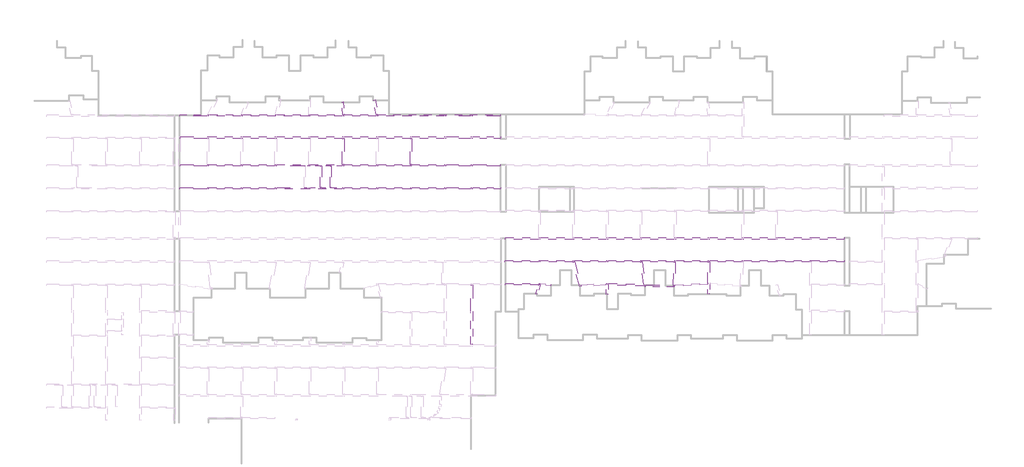
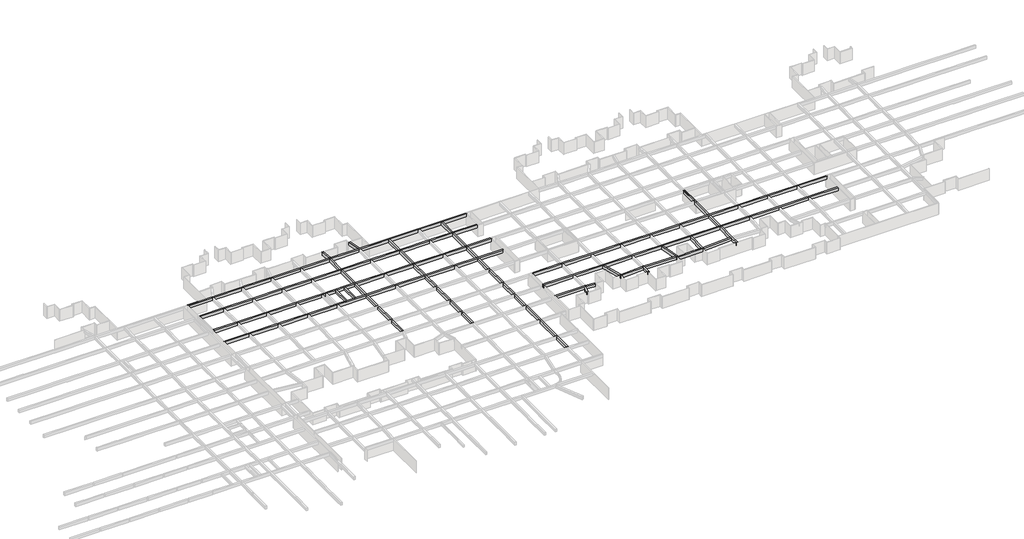
# One storey, part 14 of 16: 25 beams.
"""IFC4 building model written with IfcOpenShell, lengths in millimetres."""

from ifc_helpers import new_model, si_unit, frame, origin, place, context, project, spatial, polyline, outline, extrude, faceted_brep, element, save

model = new_model("IFC4")

# Units and contexts
model_context = context("Model", 3, world=origin())
ifc_project = project(units=[si_unit("LENGTHUNIT", "METRE", prefix="MILLI")], contexts=[model_context])

# Site, building, storey
site = spatial("IfcSite", under=ifc_project)
building = spatial("IfcBuilding", under=site)
storey = spatial("IfcBuildingStorey", under=building, Name="户型图", Elevation=0.0)

# Beams
placement = place(None, origin())
element("IfcBeam", 1, ObjectType="混凝土 - 矩形梁 : KL_beam", at=placement, inside=storey, context=model_context, shape_type="Brep", body=[
    faceted_brep([(332003.757676, -132296.8999905, 3300.0), (332003.757676, -132696.8999905, 3300.0), (332003.757676, -132696.8999905, 2500.0), (332003.757676, -132296.8999905, 2500.0), (256203.757676, -132296.8999905, 3300.0), (256203.757676, -132296.8999905, 2500.0), (256203.757676, -132696.8999905, 2500.0), (256203.757676, -132696.8999905, 3300.0), (303083.9231733, -132296.8999905, 3300.0), (302676.4364954, -132296.8999905, 3300.0), (295182.986598, -132296.8999905, 3300.0), (294781.458663, -132296.8999905, 3300.0), (287099.7203632, -132296.8999905, 3300.0), (286699.7203632, -132296.8999905, 3300.0), (279255.0563689, -132296.8999905, 3300.0), (278842.8109172, -132296.8999905, 3300.0), (271220.3376586, -132296.8999905, 3300.0), (270785.7935076, -132296.8999905, 3300.0), (263349.1220942, -132296.8999905, 3300.0), (262900.1915992, -132296.8999905, 3300.0), (262755.329592, -132696.8999905, 3300.0), (263155.329592, -132696.8999905, 3300.0), (270718.1706199, -132696.8999905, 3300.0), (271118.1706199, -132696.8999905, 3300.0), (286699.7203632, -132696.8999905, 3300.0), (287099.7203632, -132696.8999905, 3300.0), (294691.573786, -132696.8999905, 3300.0), (295091.573786, -132696.8999905, 3300.0), (302719.0558962, -132696.8999905, 3300.0), (303119.0558962, -132696.8999905, 3300.0), (310675.2880408, -132696.8999905, 3300.0), (311075.2880408, -132696.8999905, 3300.0), (318775.2880408, -132696.8999905, 3300.0), (319175.2880408, -132696.8999905, 3300.0), (325052.9173169, -132696.8999905, 3300.0), (325452.9173169, -132696.8999905, 3300.0), (262755.329592, -132696.8999905, 2500.0), (263155.329592, -132696.8999905, 2500.0), (270718.1706199, -132696.8999905, 2500.0), (271118.1706199, -132696.8999905, 2500.0), (286699.7203632, -132696.8999905, 2500.0), (287099.7203632, -132696.8999905, 2500.0), (294691.573786, -132696.8999905, 2500.0), (295091.573786, -132696.8999905, 2500.0), (302719.0558962, -132696.8999905, 2500.0), (303119.0558962, -132696.8999905, 2500.0), (310675.2880408, -132696.8999905, 2500.0), (311075.2880408, -132696.8999905, 2500.0), (318775.2880408, -132696.8999905, 2500.0), (319175.2880408, -132696.8999905, 2500.0), (325052.9173169, -132696.8999905, 2500.0), (325452.9173169, -132696.8999905, 2500.0), (262900.1915992, -132296.8999905, 2500.0), (263349.1220942, -132296.8999905, 2500.0), (270785.7935076, -132296.8999905, 2500.0), (271220.3376586, -132296.8999905, 2500.0), (278842.8109172, -132296.8999905, 2500.0), (279255.0563689, -132296.8999905, 2500.0), (286699.7203632, -132296.8999905, 2500.0), (287099.7203632, -132296.8999905, 2500.0), (294781.458663, -132296.8999905, 2500.0), (295182.986598, -132296.8999905, 2500.0), (302676.4364954, -132296.8999905, 2500.0), (303083.9231733, -132296.8999905, 2500.0)], [[[0, 1, 2, 3]], [[4, 5, 6, 7]], [[1, 0, 8, 9, 10, 11, 12, 13, 14, 15, 16, 17, 18, 19, 4, 7, 20, 21, 22, 23, 24, 25, 26, 27, 28, 29, 30, 31, 32, 33, 34, 35]], [[2, 1, 35, 34, 33, 32, 31, 30, 29, 28, 27, 26, 25, 24, 23, 22, 21, 20, 7, 6, 36, 37, 38, 39, 40, 41, 42, 43, 44, 45, 46, 47, 48, 49, 50, 51]], [[3, 2, 51, 50, 49, 48, 47, 46, 45, 44, 43, 42, 41, 40, 39, 38, 37, 36, 6, 5, 52, 53, 54, 55, 56, 57, 58, 59, 60, 61, 62, 63]], [[0, 3, 63, 62, 61, 60, 59, 58, 57, 56, 55, 54, 53, 52, 5, 4, 19, 18, 17, 16, 15, 14, 13, 12, 11, 10, 9, 8]]]),
])
element("IfcBeam", 2, ObjectType="混凝土 - 矩形梁 : KL_beam", at=placement, inside=storey, context=model_context, shape_type="SweptSolid", body=[
    extrude(outline(polyline([(294521.5830468, -129326.5081051), (294920.060926, -129291.645808), (295182.986598, -132296.8999905), (294781.458663, -132296.8999905), (294521.5830468, -129326.5081051)])), frame((0.0, 0.0, 2500.0), z_axis=(0.0, 0.0, 1.0), x_axis=(1.0, 0.0, 0.0)), (0.0, 0.0, 1.0), 800.0),
])
element("IfcBeam", 3, ObjectType="混凝土 - 矩形梁 : KL_beam", at=placement, inside=storey, context=model_context, shape_type="SweptSolid", body=[
    extrude(outline(polyline([(302016.7371766, -128903.0412108), (302409.38805, -128826.7176126), (303083.9231733, -132296.8999905), (302676.4364954, -132296.8999905), (302016.7371766, -128903.0412108)])), frame((0.0, 0.0, 2500.0), z_axis=(0.0, 0.0, 1.0), x_axis=(1.0, 0.0, 0.0)), (0.0, 0.0, 1.0), 800.0),
])
element("IfcBeam", 4, ObjectType="混凝土 - 矩形梁 : KL_beam", at=placement, inside=storey, context=model_context, shape_type="Brep", body=[
    faceted_brep([(332103.757676, -137565.7214763, 3300.0), (332103.757676, -137965.7214763, 3300.0), (332103.757676, -137965.7214763, 2500.0), (332103.757676, -137565.7214763, 2500.0), (325452.9173169, -137565.7214763, 3300.0), (325052.9173169, -137565.7214763, 3300.0), (319175.2880408, -137565.7214763, 3300.0), (318775.2880408, -137565.7214763, 3300.0), (311075.2880408, -137565.7214763, 3300.0), (310675.2880408, -137565.7214763, 3300.0), (303119.0558962, -137565.7214763, 3300.0), (302719.0558962, -137565.7214763, 3300.0), (295091.573786, -137565.7214763, 3300.0), (294691.573786, -137565.7214763, 3300.0), (287099.7203632, -137565.7214763, 3300.0), (286699.7203632, -137565.7214763, 3300.0), (279139.6845219, -137565.7214763, 3300.0), (278739.6845219, -137565.7214763, 3300.0), (271118.1706199, -137565.7214763, 3300.0), (270718.1706199, -137565.7214763, 3300.0), (263155.329592, -137565.7214763, 3300.0), (262755.329592, -137565.7214763, 3300.0), (256403.757676, -137565.7214763, 3300.0), (256403.757676, -137965.7214763, 3300.0), (262755.329592, -137965.7214763, 3300.0), (263155.329592, -137965.7214763, 3300.0), (270718.1706199, -137965.7214763, 3300.0), (271118.1706199, -137965.7214763, 3300.0), (278739.6845219, -137965.7214763, 3300.0), (279139.6845219, -137965.7214763, 3300.0), (286699.7203632, -137965.7214763, 3300.0), (287099.7203632, -137965.7214763, 3300.0), (294691.573786, -137965.7214763, 3300.0), (295091.573786, -137965.7214763, 3300.0), (302719.0558962, -137965.7214763, 3300.0), (303119.0558962, -137965.7214763, 3300.0), (310675.2880408, -137965.7214763, 3300.0), (311075.2880408, -137965.7214763, 3300.0), (318775.2880408, -137965.7214763, 3300.0), (319175.2880408, -137965.7214763, 3300.0), (325052.9173169, -137965.7214763, 3300.0), (325452.9173169, -137965.7214763, 3300.0), (256403.757676, -137965.7214763, 2500.0), (262755.329592, -137965.7214763, 2500.0), (263155.329592, -137965.7214763, 2500.0), (270718.1706199, -137965.7214763, 2500.0), (271118.1706199, -137965.7214763, 2500.0), (278739.6845219, -137965.7214763, 2500.0), (279139.6845219, -137965.7214763, 2500.0), (286699.7203632, -137965.7214763, 2500.0), (287099.7203632, -137965.7214763, 2500.0), (294691.573786, -137965.7214763, 2500.0), (295091.573786, -137965.7214763, 2500.0), (302719.0558962, -137965.7214763, 2500.0), (303119.0558962, -137965.7214763, 2500.0), (310675.2880408, -137965.7214763, 2500.0), (311075.2880408, -137965.7214763, 2500.0), (318775.2880408, -137965.7214763, 2500.0), (319175.2880408, -137965.7214763, 2500.0), (325052.9173169, -137965.7214763, 2500.0), (325452.9173169, -137965.7214763, 2500.0), (256403.757676, -137565.7214763, 2500.0), (262755.329592, -137565.7214763, 2500.0), (263155.329592, -137565.7214763, 2500.0), (270718.1706199, -137565.7214763, 2500.0), (271118.1706199, -137565.7214763, 2500.0), (278739.6845219, -137565.7214763, 2500.0), (279139.6845219, -137565.7214763, 2500.0), (286699.7203632, -137565.7214763, 2500.0), (287099.7203632, -137565.7214763, 2500.0), (294691.573786, -137565.7214763, 2500.0), (295091.573786, -137565.7214763, 2500.0), (302719.0558962, -137565.7214763, 2500.0), (303119.0558962, -137565.7214763, 2500.0), (310675.2880408, -137565.7214763, 2500.0), (311075.2880408, -137565.7214763, 2500.0), (318775.2880408, -137565.7214763, 2500.0), (319175.2880408, -137565.7214763, 2500.0), (325052.9173169, -137565.7214763, 2500.0), (325452.9173169, -137565.7214763, 2500.0)], [[[0, 1, 2, 3]], [[1, 0, 4, 5, 6, 7, 8, 9, 10, 11, 12, 13, 14, 15, 16, 17, 18, 19, 20, 21, 22, 23, 24, 25, 26, 27, 28, 29, 30, 31, 32, 33, 34, 35, 36, 37, 38, 39, 40, 41]], [[2, 1, 41, 40, 39, 38, 37, 36, 35, 34, 33, 32, 31, 30, 29, 28, 27, 26, 25, 24, 23, 42, 43, 44, 45, 46, 47, 48, 49, 50, 51, 52, 53, 54, 55, 56, 57, 58, 59, 60]], [[3, 2, 60, 59, 58, 57, 56, 55, 54, 53, 52, 51, 50, 49, 48, 47, 46, 45, 44, 43, 42, 61, 62, 63, 64, 65, 66, 67, 68, 69, 70, 71, 72, 73, 74, 75, 76, 77, 78, 79]], [[0, 3, 79, 78, 77, 76, 75, 74, 73, 72, 71, 70, 69, 68, 67, 66, 65, 64, 63, 62, 61, 22, 21, 20, 19, 18, 17, 16, 15, 14, 13, 12, 11, 10, 9, 8, 7, 6, 5, 4]], [[23, 22, 61, 42]]]),
])
element("IfcBeam", 5, ObjectType="混凝土 - 矩形梁 : KL_beam", at=placement, inside=storey, context=model_context, shape_type="Brep", body=[
    faceted_brep([(332003.757676, -144125.7214763, 3300.0), (332003.757676, -144525.7214763, 3300.0), (332003.757676, -144525.7214763, 2500.0), (332003.757676, -144125.7214763, 2500.0), (325452.9173169, -144125.7214763, 3300.0), (325052.9173169, -144125.7214763, 3300.0), (319175.2880408, -144125.7214763, 3300.0), (318775.2880408, -144125.7214763, 3300.0), (311075.2880408, -144125.7214763, 3300.0), (310675.2880408, -144125.7214763, 3300.0), (303119.0558962, -144125.7214763, 3300.0), (302719.0558962, -144125.7214763, 3300.0), (295091.573786, -144125.7214763, 3300.0), (294691.573786, -144125.7214763, 3300.0), (287099.7203632, -144125.7214763, 3300.0), (286699.7203632, -144125.7214763, 3300.0), (279139.6845219, -144125.7214763, 3300.0), (278739.6845219, -144125.7214763, 3300.0), (271118.1706199, -144125.7214763, 3300.0), (270718.1706199, -144125.7214763, 3300.0), (263155.329592, -144125.7214763, 3300.0), (262755.329592, -144125.7214763, 3300.0), (256403.757676, -144125.7214763, 3300.0), (256403.757676, -144525.7214763, 3300.0), (262755.329592, -144525.7214763, 3300.0), (263155.329592, -144525.7214763, 3300.0), (270718.1706199, -144525.7214763, 3300.0), (271118.1706199, -144525.7214763, 3300.0), (278739.6845219, -144525.7214763, 3300.0), (279139.6845219, -144525.7214763, 3300.0), (285649.7203632, -144525.7214763, 3300.0), (285949.7203632, -144525.7214763, 3300.0), (286699.7203632, -144525.7214763, 3300.0), (287099.7203632, -144525.7214763, 3300.0), (289449.7203632, -144525.7214763, 3300.0), (289749.7203632, -144525.7214763, 3300.0), (291749.7203632, -144525.7214763, 3300.0), (292049.7203632, -144525.7214763, 3300.0), (294691.573786, -144525.7214763, 3300.0), (295091.573786, -144525.7214763, 3300.0), (302719.0558962, -144525.7214763, 3300.0), (303119.0558962, -144525.7214763, 3300.0), (310675.2880408, -144525.7214763, 3300.0), (311075.2880408, -144525.7214763, 3300.0), (318775.2880408, -144525.7214763, 3300.0), (319175.2880408, -144525.7214763, 3300.0), (325052.9173169, -144525.7214763, 3300.0), (325452.9173169, -144525.7214763, 3300.0), (256403.757676, -144525.7214763, 2500.0), (262755.329592, -144525.7214763, 2500.0), (263155.329592, -144525.7214763, 2500.0), (270718.1706199, -144525.7214763, 2500.0), (271118.1706199, -144525.7214763, 2500.0), (278739.6845219, -144525.7214763, 2500.0), (279139.6845219, -144525.7214763, 2500.0), (286699.7203632, -144525.7214763, 2500.0), (287099.7203632, -144525.7214763, 2500.0), (294691.573786, -144525.7214763, 2500.0), (295091.573786, -144525.7214763, 2500.0), (302719.0558962, -144525.7214763, 2500.0), (303119.0558962, -144525.7214763, 2500.0), (310675.2880408, -144525.7214763, 2500.0), (311075.2880408, -144525.7214763, 2500.0), (318775.2880408, -144525.7214763, 2500.0), (319175.2880408, -144525.7214763, 2500.0), (325052.9173169, -144525.7214763, 2500.0), (325452.9173169, -144525.7214763, 2500.0), (256403.757676, -144125.7214763, 2500.0), (262755.329592, -144125.7214763, 2500.0), (263155.329592, -144125.7214763, 2500.0), (270718.1706199, -144125.7214763, 2500.0), (271118.1706199, -144125.7214763, 2500.0), (278739.6845219, -144125.7214763, 2500.0), (279139.6845219, -144125.7214763, 2500.0), (286699.7203632, -144125.7214763, 2500.0), (287099.7203632, -144125.7214763, 2500.0), (294691.573786, -144125.7214763, 2500.0), (295091.573786, -144125.7214763, 2500.0), (302719.0558962, -144125.7214763, 2500.0), (303119.0558962, -144125.7214763, 2500.0), (310675.2880408, -144125.7214763, 2500.0), (311075.2880408, -144125.7214763, 2500.0), (318775.2880408, -144125.7214763, 2500.0), (319175.2880408, -144125.7214763, 2500.0), (325052.9173169, -144125.7214763, 2500.0), (325452.9173169, -144125.7214763, 2500.0)], [[[0, 1, 2, 3]], [[1, 0, 4, 5, 6, 7, 8, 9, 10, 11, 12, 13, 14, 15, 16, 17, 18, 19, 20, 21, 22, 23, 24, 25, 26, 27, 28, 29, 30, 31, 32, 33, 34, 35, 36, 37, 38, 39, 40, 41, 42, 43, 44, 45, 46, 47]], [[2, 1, 47, 46, 45, 44, 43, 42, 41, 40, 39, 38, 37, 36, 35, 34, 33, 32, 31, 30, 29, 28, 27, 26, 25, 24, 23, 48, 49, 50, 51, 52, 53, 54, 55, 56, 57, 58, 59, 60, 61, 62, 63, 64, 65, 66]], [[3, 2, 66, 65, 64, 63, 62, 61, 60, 59, 58, 57, 56, 55, 54, 53, 52, 51, 50, 49, 48, 67, 68, 69, 70, 71, 72, 73, 74, 75, 76, 77, 78, 79, 80, 81, 82, 83, 84, 85]], [[0, 3, 85, 84, 83, 82, 81, 80, 79, 78, 77, 76, 75, 74, 73, 72, 71, 70, 69, 68, 67, 22, 21, 20, 19, 18, 17, 16, 15, 14, 13, 12, 11, 10, 9, 8, 7, 6, 5, 4]], [[23, 22, 67, 48]]]),
])
element("IfcBeam", 6, ObjectType="混凝土 - 矩形梁 : KL_beam", at=placement, inside=storey, context=model_context, shape_type="Brep", body=[
    faceted_brep([(332103.757676, -149525.7214763, 3300.0), (332103.757676, -149925.7214763, 3300.0), (332103.757676, -149925.7214763, 2500.0), (332103.757676, -149525.7214763, 2500.0), (256203.757676, -149525.7214763, 3300.0), (256203.757676, -149525.7214763, 2500.0), (256203.757676, -149925.7214763, 2500.0), (256203.757676, -149925.7214763, 3300.0), (325452.9173169, -149525.7214763, 3300.0), (325052.9173169, -149525.7214763, 3300.0), (319175.2880408, -149525.7214763, 3300.0), (318775.2880408, -149525.7214763, 3300.0), (311075.2880408, -149525.7214763, 3300.0), (310675.2880408, -149525.7214763, 3300.0), (303119.0558962, -149525.7214763, 3300.0), (302719.0558962, -149525.7214763, 3300.0), (295091.573786, -149525.7214763, 3300.0), (294691.573786, -149525.7214763, 3300.0), (292049.7203632, -149525.7214763, 3300.0), (291749.7203632, -149525.7214763, 3300.0), (289749.7203632, -149525.7214763, 3300.0), (289449.7203632, -149525.7214763, 3300.0), (287099.7203632, -149525.7214763, 3300.0), (286699.7203632, -149525.7214763, 3300.0), (285949.7203632, -149525.7214763, 3300.0), (285649.7203632, -149525.7214763, 3300.0), (279139.6845219, -149525.7214763, 3300.0), (278739.6845219, -149525.7214763, 3300.0), (271118.1706199, -149525.7214763, 3300.0), (270718.1706199, -149525.7214763, 3300.0), (263155.329592, -149525.7214763, 3300.0), (262755.329592, -149525.7214763, 3300.0), (262755.329592, -149925.7214763, 3300.0), (263155.329592, -149925.7214763, 3300.0), (270718.1706199, -149925.7214763, 3300.0), (271118.1706199, -149925.7214763, 3300.0), (278739.6845219, -149925.7214763, 3300.0), (279139.6845219, -149925.7214763, 3300.0), (286699.7203632, -149925.7214763, 3300.0), (287099.7203632, -149925.7214763, 3300.0), (294691.573786, -149925.7214763, 3300.0), (295091.573786, -149925.7214763, 3300.0), (302719.0558962, -149925.7214763, 3300.0), (303119.0558962, -149925.7214763, 3300.0), (310675.2880408, -149925.7214763, 3300.0), (311075.2880408, -149925.7214763, 3300.0), (318775.2880408, -149925.7214763, 3300.0), (319175.2880408, -149925.7214763, 3300.0), (325052.9173169, -149925.7214763, 3300.0), (325452.9173169, -149925.7214763, 3300.0), (262755.329592, -149925.7214763, 2500.0), (263155.329592, -149925.7214763, 2500.0), (270718.1706199, -149925.7214763, 2500.0), (271118.1706199, -149925.7214763, 2500.0), (278739.6845219, -149925.7214763, 2500.0), (279139.6845219, -149925.7214763, 2500.0), (286699.7203632, -149925.7214763, 2500.0), (287099.7203632, -149925.7214763, 2500.0), (294691.573786, -149925.7214763, 2500.0), (295091.573786, -149925.7214763, 2500.0), (302719.0558962, -149925.7214763, 2500.0), (303119.0558962, -149925.7214763, 2500.0), (310675.2880408, -149925.7214763, 2500.0), (311075.2880408, -149925.7214763, 2500.0), (318775.2880408, -149925.7214763, 2500.0), (319175.2880408, -149925.7214763, 2500.0), (325052.9173169, -149925.7214763, 2500.0), (325452.9173169, -149925.7214763, 2500.0), (262755.329592, -149525.7214763, 2500.0), (263155.329592, -149525.7214763, 2500.0), (270718.1706199, -149525.7214763, 2500.0), (271118.1706199, -149525.7214763, 2500.0), (278739.6845219, -149525.7214763, 2500.0), (279139.6845219, -149525.7214763, 2500.0), (286699.7203632, -149525.7214763, 2500.0), (287099.7203632, -149525.7214763, 2500.0), (294691.573786, -149525.7214763, 2500.0), (295091.573786, -149525.7214763, 2500.0), (302719.0558962, -149525.7214763, 2500.0), (303119.0558962, -149525.7214763, 2500.0), (310675.2880408, -149525.7214763, 2500.0), (311075.2880408, -149525.7214763, 2500.0), (318775.2880408, -149525.7214763, 2500.0), (319175.2880408, -149525.7214763, 2500.0), (325052.9173169, -149525.7214763, 2500.0), (325452.9173169, -149525.7214763, 2500.0)], [[[0, 1, 2, 3]], [[4, 5, 6, 7]], [[1, 0, 8, 9, 10, 11, 12, 13, 14, 15, 16, 17, 18, 19, 20, 21, 22, 23, 24, 25, 26, 27, 28, 29, 30, 31, 4, 7, 32, 33, 34, 35, 36, 37, 38, 39, 40, 41, 42, 43, 44, 45, 46, 47, 48, 49]], [[2, 1, 49, 48, 47, 46, 45, 44, 43, 42, 41, 40, 39, 38, 37, 36, 35, 34, 33, 32, 7, 6, 50, 51, 52, 53, 54, 55, 56, 57, 58, 59, 60, 61, 62, 63, 64, 65, 66, 67]], [[3, 2, 67, 66, 65, 64, 63, 62, 61, 60, 59, 58, 57, 56, 55, 54, 53, 52, 51, 50, 6, 5, 68, 69, 70, 71, 72, 73, 74, 75, 76, 77, 78, 79, 80, 81, 82, 83, 84, 85]], [[0, 3, 85, 84, 83, 82, 81, 80, 79, 78, 77, 76, 75, 74, 73, 72, 71, 70, 69, 68, 5, 4, 31, 30, 29, 28, 27, 26, 25, 24, 23, 22, 21, 20, 19, 18, 17, 16, 15, 14, 13, 12, 11, 10, 9, 8]]]),
])
element("IfcBeam", 7, ObjectType="混凝土 - 矩形梁 : KL_beam", at=placement, inside=storey, context=model_context, shape_type="SweptSolid", body=[
    extrude(outline(polyline([(295091.573786, -166823.3600959), (294691.573786, -166823.3600959), (294691.573786, -161826.0461868), (295091.573786, -161826.0461868), (295091.573786, -166823.3600959)])), frame((0.0, 0.0, 2500.0), z_axis=(0.0, 0.0, 1.0), x_axis=(1.0, 0.0, 0.0)), (0.0, 0.0, 1.0), 800.0),
    extrude(outline(polyline([(294691.573786, -132696.8999905), (295091.573786, -132696.8999905), (295091.573786, -137565.7214763), (294691.573786, -137565.7214763), (294691.573786, -132696.8999905)])), frame((0.0, 0.0, 2500.0), z_axis=(0.0, 0.0, 1.0), x_axis=(1.0, 0.0, 0.0)), (0.0, 0.0, 1.0), 800.0),
    extrude(outline(polyline([(294691.573786, -137965.7214763), (295091.573786, -137965.7214763), (295091.573786, -144125.7214763), (294691.573786, -144125.7214763), (294691.573786, -137965.7214763)])), frame((0.0, 0.0, 2500.0), z_axis=(0.0, 0.0, 1.0), x_axis=(1.0, 0.0, 0.0)), (0.0, 0.0, 1.0), 800.0),
    extrude(outline(polyline([(294691.573786, -144525.7214763), (295091.573786, -144525.7214763), (295091.573786, -149525.7214763), (294691.573786, -149525.7214763), (294691.573786, -144525.7214763)])), frame((0.0, 0.0, 2500.0), z_axis=(0.0, 0.0, 1.0), x_axis=(1.0, 0.0, 0.0)), (0.0, 0.0, 1.0), 800.0),
    extrude(outline(polyline([(294691.573786, -149925.7214763), (295091.573786, -149925.7214763), (295091.573786, -154958.1403142), (294691.573786, -154958.1403142), (294691.573786, -149925.7214763)])), frame((0.0, 0.0, 2500.0), z_axis=(0.0, 0.0, 1.0), x_axis=(1.0, 0.0, 0.0)), (0.0, 0.0, 1.0), 800.0),
    extrude(outline(polyline([(294691.573786, -155358.1403142), (295091.573786, -155358.1403142), (295091.573786, -161426.0461868), (294691.573786, -161426.0461868), (294691.573786, -155358.1403142)])), frame((0.0, 0.0, 2500.0), z_axis=(0.0, 0.0, 1.0), x_axis=(1.0, 0.0, 0.0)), (0.0, 0.0, 1.0), 800.0),
])
element("IfcBeam", 8, ObjectType="混凝土 - 矩形梁 : KL_beam", at=placement, inside=storey, context=model_context, shape_type="SweptSolid", body=[
    extrude(outline(polyline([(311075.2880408, -172196.8999905), (310675.2880408, -172196.8999905), (310675.2880408, -167223.3600959), (311075.2880408, -167223.3600959), (311075.2880408, -172196.8999905)])), frame((0.0, 0.0, 2500.0), z_axis=(0.0, 0.0, 1.0), x_axis=(1.0, 0.0, 0.0)), (0.0, 0.0, 1.0), 800.0),
    extrude(outline(polyline([(310675.2880408, -132696.8999905), (311075.2880408, -132696.8999905), (311075.2880408, -137565.7214763), (310675.2880408, -137565.7214763), (310675.2880408, -132696.8999905)])), frame((0.0, 0.0, 2500.0), z_axis=(0.0, 0.0, 1.0), x_axis=(1.0, 0.0, 0.0)), (0.0, 0.0, 1.0), 800.0),
    extrude(outline(polyline([(310675.2880408, -137965.7214763), (311075.2880408, -137965.7214763), (311075.2880408, -144125.7214763), (310675.2880408, -144125.7214763), (310675.2880408, -137965.7214763)])), frame((0.0, 0.0, 2500.0), z_axis=(0.0, 0.0, 1.0), x_axis=(1.0, 0.0, 0.0)), (0.0, 0.0, 1.0), 800.0),
    extrude(outline(polyline([(310675.2880408, -144525.7214763), (311075.2880408, -144525.7214763), (311075.2880408, -149525.7214763), (310675.2880408, -149525.7214763), (310675.2880408, -144525.7214763)])), frame((0.0, 0.0, 2500.0), z_axis=(0.0, 0.0, 1.0), x_axis=(1.0, 0.0, 0.0)), (0.0, 0.0, 1.0), 800.0),
    extrude(outline(polyline([(310675.2880408, -149925.7214763), (311075.2880408, -149925.7214763), (311075.2880408, -154958.1403142), (310675.2880408, -154958.1403142), (310675.2880408, -149925.7214763)])), frame((0.0, 0.0, 2500.0), z_axis=(0.0, 0.0, 1.0), x_axis=(1.0, 0.0, 0.0)), (0.0, 0.0, 1.0), 800.0),
    extrude(outline(polyline([(310675.2880408, -155358.1403142), (311075.2880408, -155358.1403142), (311075.2880408, -161426.0461868), (310675.2880408, -161426.0461868), (310675.2880408, -155358.1403142)])), frame((0.0, 0.0, 2500.0), z_axis=(0.0, 0.0, 1.0), x_axis=(1.0, 0.0, 0.0)), (0.0, 0.0, 1.0), 800.0),
    extrude(outline(polyline([(310675.2880408, -161826.0461868), (311075.2880408, -161826.0461868), (311075.2880408, -166823.3600959), (310675.2880408, -166823.3600959), (310675.2880408, -161826.0461868)])), frame((0.0, 0.0, 2500.0), z_axis=(0.0, 0.0, 1.0), x_axis=(1.0, 0.0, 0.0)), (0.0, 0.0, 1.0), 800.0),
])
element("IfcBeam", 9, ObjectType="混凝土 - 矩形梁 : KL_beam", at=placement, inside=storey, context=model_context, shape_type="Brep", body=[
    faceted_brep([(325052.9173169, -191962.1668684, 3300.0), (325452.9173169, -191962.1668684, 3300.0), (325452.9173169, -187062.1668684, 3300.0), (325052.9173169, -187062.1668684, 3300.0), (325452.9173169, -191962.1668684, 2500.0), (325452.9173169, -187062.1668684, 2500.0), (325052.9173169, -191962.1668684, 2500.0), (325052.9173169, -187062.1668684, 2500.0)], [[[0, 1, 2, 3]], [[1, 4, 5, 2]], [[4, 6, 7, 5]], [[6, 0, 3, 7]], [[1, 0, 6, 4]], [[3, 2, 5, 7]]]),
    faceted_brep([(325052.9173169, -132696.8999905, 3300.0), (325452.9173169, -132696.8999905, 3300.0), (325452.9173169, -132696.8999905, 2500.0), (325052.9173169, -132696.8999905, 2500.0), (325452.9173169, -137565.7214763, 3300.0), (325052.9173169, -137565.7214763, 3300.0), (325052.9173169, -137565.7214763, 2500.0), (325452.9173169, -137565.7214763, 2500.0)], [[[0, 1, 2, 3]], [[4, 5, 6, 7]], [[1, 0, 5, 4]], [[2, 1, 4, 7]], [[3, 2, 7, 6]], [[0, 3, 6, 5]]]),
    faceted_brep([(325052.9173169, -137965.7214763, 3300.0), (325452.9173169, -137965.7214763, 3300.0), (325452.9173169, -137965.7214763, 2500.0), (325052.9173169, -137965.7214763, 2500.0), (325452.9173169, -144125.7214763, 3300.0), (325052.9173169, -144125.7214763, 3300.0), (325052.9173169, -144125.7214763, 2500.0), (325452.9173169, -144125.7214763, 2500.0)], [[[0, 1, 2, 3]], [[4, 5, 6, 7]], [[1, 0, 5, 4]], [[2, 1, 4, 7]], [[3, 2, 7, 6]], [[0, 3, 6, 5]]]),
    faceted_brep([(325052.9173169, -144525.7214763, 3300.0), (325452.9173169, -144525.7214763, 3300.0), (325452.9173169, -144525.7214763, 2500.0), (325052.9173169, -144525.7214763, 2500.0), (325452.9173169, -149525.7214763, 3300.0), (325052.9173169, -149525.7214763, 3300.0), (325052.9173169, -149525.7214763, 2500.0), (325452.9173169, -149525.7214763, 2500.0)], [[[0, 1, 2, 3]], [[4, 5, 6, 7]], [[1, 0, 5, 4]], [[2, 1, 4, 7]], [[3, 2, 7, 6]], [[0, 3, 6, 5]]]),
    faceted_brep([(325052.9173169, -149925.7214763, 3300.0), (325452.9173169, -149925.7214763, 3300.0), (325452.9173169, -149925.7214763, 2500.0), (325052.9173169, -149925.7214763, 2500.0), (325452.9173169, -154958.1403142, 3300.0), (325052.9173169, -154958.1403142, 3300.0), (325052.9173169, -154958.1403142, 2500.0), (325452.9173169, -154958.1403142, 2500.0)], [[[0, 1, 2, 3]], [[4, 5, 6, 7]], [[1, 0, 5, 4]], [[2, 1, 4, 7]], [[3, 2, 7, 6]], [[0, 3, 6, 5]]]),
    faceted_brep([(325052.9173169, -155358.1403142, 3300.0), (325452.9173169, -155358.1403142, 3300.0), (325452.9173169, -155358.1403142, 2500.0), (325052.9173169, -155358.1403142, 2500.0), (325452.9173169, -161426.0461868, 3300.0), (325052.9173169, -161426.0461868, 3300.0), (325052.9173169, -161426.0461868, 2500.0), (325452.9173169, -161426.0461868, 2500.0)], [[[0, 1, 2, 3]], [[4, 5, 6, 7]], [[1, 0, 5, 4]], [[2, 1, 4, 7]], [[3, 2, 7, 6]], [[0, 3, 6, 5]]]),
    faceted_brep([(325052.9173169, -161826.0461868, 3300.0), (325452.9173169, -161826.0461868, 3300.0), (325452.9173169, -161826.0461868, 2500.0), (325052.9173169, -161826.0461868, 2500.0), (325452.9173169, -166823.3600959, 3300.0), (325052.9173169, -166823.3600959, 3300.0), (325052.9173169, -166823.3600959, 2500.0), (325452.9173169, -166823.3600959, 2500.0)], [[[0, 1, 2, 3]], [[4, 5, 6, 7]], [[1, 0, 5, 4]], [[2, 1, 4, 7]], [[3, 2, 7, 6]], [[0, 3, 6, 5]]]),
    faceted_brep([(325052.9173169, -167223.3600959, 3300.0), (325452.9173169, -167223.3600959, 3300.0), (325452.9173169, -167223.3600959, 2500.0), (325052.9173169, -167223.3600959, 2500.0), (325052.9173169, -172196.8999905, 3300.0), (325452.9173169, -172196.8999905, 3300.0), (325452.9173169, -172196.8999905, 2500.0), (325052.9173169, -172196.8999905, 2500.0)], [[[0, 1, 2, 3]], [[1, 0, 4, 5]], [[2, 1, 5, 6]], [[3, 2, 6, 7]], [[0, 3, 7, 4]], [[5, 4, 7, 6]]]),
    faceted_brep([(325452.9173169, -186662.1668684, 3300.0), (325052.9173169, -186662.1668684, 3300.0), (325052.9173169, -186662.1668684, 2500.0), (325452.9173169, -186662.1668684, 2500.0), (325052.9173169, -172596.8999905, 3300.0), (325452.9173169, -172596.8999905, 3300.0), (325452.9173169, -172596.8999905, 2500.0), (325052.9173169, -172596.8999905, 2500.0), (325452.9173169, -179243.9042946, 3300.0), (325452.9173169, -178843.9042946, 3300.0), (325052.9173169, -178843.9042946, 3300.0), (325052.9173169, -179243.9042946, 3300.0), (325452.9173169, -179243.9042946, 2500.0), (325452.9173169, -178843.9042946, 2500.0), (325052.9173169, -179243.9042946, 2500.0), (325052.9173169, -178843.9042946, 2500.0)], [[[0, 1, 2, 3]], [[4, 5, 6, 7]], [[1, 0, 8, 9, 5, 4, 10, 11]], [[0, 3, 12, 13, 6, 5, 9, 8]], [[3, 2, 14, 15, 7, 6, 13, 12]], [[2, 1, 11, 10, 4, 7, 15, 14]]]),
])
element("IfcBeam", 10, ObjectType="混凝土 - 矩形梁 : KL_beam", at=placement, inside=storey, context=model_context, shape_type="Brep", body=[
    faceted_brep([(413278.7576761, -161426.0461868, 3300.0), (413278.7576761, -161826.0461868, 3300.0), (413278.7576761, -161826.0461868, 2500.0), (413278.7576761, -161426.0461868, 2500.0), (333153.7576761, -161426.0461868, 3300.0), (333153.7576761, -161426.0461868, 2500.0), (333153.7576761, -161826.0461868, 2500.0), (333153.7576761, -161826.0461868, 3300.0), (405478.7576761, -161426.0461868, 3300.0), (405078.7576761, -161426.0461868, 3300.0), (397425.7298502, -161426.0461868, 3300.0), (397025.7298502, -161426.0461868, 3300.0), (389433.5747738, -161426.0461868, 3300.0), (389033.5747738, -161426.0461868, 3300.0), (381435.9353884, -161426.0461868, 3300.0), (381035.9353884, -161426.0461868, 3300.0), (373507.5350349, -161426.0461868, 3300.0), (373107.5350349, -161426.0461868, 3300.0), (365445.2144882, -161426.0461868, 3300.0), (365045.2144882, -161426.0461868, 3300.0), (357429.5901603, -161426.0461868, 3300.0), (357029.5901603, -161426.0461868, 3300.0), (349446.5285699, -161426.0461868, 3300.0), (349046.5285699, -161426.0461868, 3300.0), (341453.7576761, -161426.0461868, 3300.0), (341053.7576761, -161426.0461868, 3300.0), (341053.7576761, -161826.0461868, 3300.0), (341453.7576761, -161826.0461868, 3300.0), (349046.5285699, -161826.0461868, 3300.0), (349446.5285699, -161826.0461868, 3300.0), (357029.5901603, -161826.0461868, 3300.0), (357429.5901603, -161826.0461868, 3300.0), (365045.2144882, -161826.0461868, 3300.0), (365445.2144882, -161826.0461868, 3300.0), (373107.5350349, -161826.0461868, 3300.0), (373507.5350349, -161826.0461868, 3300.0), (381035.9353884, -161826.0461868, 3300.0), (381435.9353884, -161826.0461868, 3300.0), (389033.5747738, -161826.0461868, 3300.0), (389433.5747738, -161826.0461868, 3300.0), (397025.7298502, -161826.0461868, 3300.0), (397425.7298502, -161826.0461868, 3300.0), (405078.7576761, -161826.0461868, 3300.0), (405478.7576761, -161826.0461868, 3300.0), (341053.7576761, -161826.0461868, 2500.0), (341453.7576761, -161826.0461868, 2500.0), (349046.5285699, -161826.0461868, 2500.0), (349446.5285699, -161826.0461868, 2500.0), (357029.5901603, -161826.0461868, 2500.0), (357429.5901603, -161826.0461868, 2500.0), (365045.2144882, -161826.0461868, 2500.0), (365445.2144882, -161826.0461868, 2500.0), (373107.5350349, -161826.0461868, 2500.0), (373507.5350349, -161826.0461868, 2500.0), (381035.9353884, -161826.0461868, 2500.0), (381435.9353884, -161826.0461868, 2500.0), (389033.5747738, -161826.0461868, 2500.0), (389433.5747738, -161826.0461868, 2500.0), (397025.7298502, -161826.0461868, 2500.0), (397425.7298502, -161826.0461868, 2500.0), (405078.7576761, -161826.0461868, 2500.0), (405478.7576761, -161826.0461868, 2500.0), (341053.7576761, -161426.0461868, 2500.0), (341453.7576761, -161426.0461868, 2500.0), (349046.5285699, -161426.0461868, 2500.0), (349446.5285699, -161426.0461868, 2500.0), (357029.5901603, -161426.0461868, 2500.0), (357429.5901603, -161426.0461868, 2500.0), (365045.2144882, -161426.0461868, 2500.0), (365445.2144882, -161426.0461868, 2500.0), (373107.5350349, -161426.0461868, 2500.0), (373507.5350349, -161426.0461868, 2500.0), (381035.9353884, -161426.0461868, 2500.0), (381435.9353884, -161426.0461868, 2500.0), (389033.5747738, -161426.0461868, 2500.0), (389433.5747738, -161426.0461868, 2500.0), (397025.7298502, -161426.0461868, 2500.0), (397425.7298502, -161426.0461868, 2500.0), (405078.7576761, -161426.0461868, 2500.0), (405478.7576761, -161426.0461868, 2500.0)], [[[0, 1, 2, 3]], [[4, 5, 6, 7]], [[1, 0, 8, 9, 10, 11, 12, 13, 14, 15, 16, 17, 18, 19, 20, 21, 22, 23, 24, 25, 4, 7, 26, 27, 28, 29, 30, 31, 32, 33, 34, 35, 36, 37, 38, 39, 40, 41, 42, 43]], [[2, 1, 43, 42, 41, 40, 39, 38, 37, 36, 35, 34, 33, 32, 31, 30, 29, 28, 27, 26, 7, 6, 44, 45, 46, 47, 48, 49, 50, 51, 52, 53, 54, 55, 56, 57, 58, 59, 60, 61]], [[3, 2, 61, 60, 59, 58, 57, 56, 55, 54, 53, 52, 51, 50, 49, 48, 47, 46, 45, 44, 6, 5, 62, 63, 64, 65, 66, 67, 68, 69, 70, 71, 72, 73, 74, 75, 76, 77, 78, 79]], [[0, 3, 79, 78, 77, 76, 75, 74, 73, 72, 71, 70, 69, 68, 67, 66, 65, 64, 63, 62, 5, 4, 25, 24, 23, 22, 21, 20, 19, 18, 17, 16, 15, 14, 13, 12, 11, 10, 9, 8]]]),
])
element("IfcBeam", 11, ObjectType="混凝土 - 矩形梁 : KL_beam", at=placement, inside=storey, context=model_context, shape_type="Brep", body=[
    faceted_brep([(413278.7576761, -166805.1471774, 3300.0), (413278.7576761, -167205.1471774, 3300.0), (413278.7576761, -167205.1471774, 2500.0), (413278.7576761, -166805.1471774, 2500.0), (333053.7576761, -166805.1471774, 3300.0), (333053.7576761, -166805.1471774, 2500.0), (333053.7576761, -167205.1471774, 2500.0), (333053.7576761, -167205.1471774, 3300.0), (405478.7576761, -166805.1471774, 3300.0), (405078.7576761, -166805.1471774, 3300.0), (397425.7298502, -166805.1471774, 3300.0), (397025.7298502, -166805.1471774, 3300.0), (389433.5747738, -166805.1471774, 3300.0), (389033.5747738, -166805.1471774, 3300.0), (381435.9353884, -166805.1471774, 3300.0), (381035.9353884, -166805.1471774, 3300.0), (373507.5350349, -166805.1471774, 3300.0), (373107.5350349, -166805.1471774, 3300.0), (365445.2144882, -166805.1471774, 3300.0), (365045.2144882, -166805.1471774, 3300.0), (357429.5901603, -166805.1471774, 3300.0), (357029.5901603, -166805.1471774, 3300.0), (349446.5285699, -166805.1471774, 3300.0), (349046.5285699, -166805.1471774, 3300.0), (341453.7576761, -166805.1471774, 3300.0), (341053.7576761, -166805.1471774, 3300.0), (341053.7576761, -167205.1471774, 3300.0), (341453.7576761, -167205.1471774, 3300.0), (349094.9105218, -167205.1471774, 3300.0), (349510.3494046, -167205.1471774, 3300.0), (357029.5901603, -167205.1471774, 3300.0), (357429.5901603, -167205.1471774, 3300.0), (365074.1284064, -167205.1471774, 3300.0), (365479.0149212, -167205.1471774, 3300.0), (372961.7518449, -167205.1471774, 3300.0), (373361.8511209, -167205.1471774, 3300.0), (381035.9353884, -167205.1471774, 3300.0), (381435.9353884, -167205.1471774, 3300.0), (389019.1010318, -167205.1471774, 3300.0), (389420.0777911, -167205.1471774, 3300.0), (397025.7298502, -167205.1471774, 3300.0), (397425.7298502, -167205.1471774, 3300.0), (405078.7576761, -167205.1471774, 3300.0), (405478.7576761, -167205.1471774, 3300.0), (341053.7576761, -167205.1471774, 2500.0), (341453.7576761, -167205.1471774, 2500.0), (349094.9105218, -167205.1471774, 2500.0), (349510.3494046, -167205.1471774, 2500.0), (357029.5901603, -167205.1471774, 2500.0), (357429.5901603, -167205.1471774, 2500.0), (365074.1284064, -167205.1471774, 2500.0), (365479.0149212, -167205.1471774, 2500.0), (372961.7518449, -167205.1471774, 2500.0), (373361.8511209, -167205.1471774, 2500.0), (381035.9353884, -167205.1471774, 2500.0), (381435.9353884, -167205.1471774, 2500.0), (389019.1010318, -167205.1471774, 2500.0), (389420.0777911, -167205.1471774, 2500.0), (397025.7298502, -167205.1471774, 2500.0), (397425.7298502, -167205.1471774, 2500.0), (405078.7576761, -167205.1471774, 2500.0), (405478.7576761, -167205.1471774, 2500.0), (341053.7576761, -166805.1471774, 2500.0), (341453.7576761, -166805.1471774, 2500.0), (349046.5285699, -166805.1471774, 2500.0), (349446.5285699, -166805.1471774, 2500.0), (357029.5901603, -166805.1471774, 2500.0), (357429.5901603, -166805.1471774, 2500.0), (365045.2144882, -166805.1471774, 2500.0), (365445.2144882, -166805.1471774, 2500.0), (373107.5350349, -166805.1471774, 2500.0), (373507.5350349, -166805.1471774, 2500.0), (381035.9353884, -166805.1471774, 2500.0), (381435.9353884, -166805.1471774, 2500.0), (389033.5747738, -166805.1471774, 2500.0), (389433.5747738, -166805.1471774, 2500.0), (397025.7298502, -166805.1471774, 2500.0), (397425.7298502, -166805.1471774, 2500.0), (405078.7576761, -166805.1471774, 2500.0), (405478.7576761, -166805.1471774, 2500.0)], [[[0, 1, 2, 3]], [[4, 5, 6, 7]], [[1, 0, 8, 9, 10, 11, 12, 13, 14, 15, 16, 17, 18, 19, 20, 21, 22, 23, 24, 25, 4, 7, 26, 27, 28, 29, 30, 31, 32, 33, 34, 35, 36, 37, 38, 39, 40, 41, 42, 43]], [[2, 1, 43, 42, 41, 40, 39, 38, 37, 36, 35, 34, 33, 32, 31, 30, 29, 28, 27, 26, 7, 6, 44, 45, 46, 47, 48, 49, 50, 51, 52, 53, 54, 55, 56, 57, 58, 59, 60, 61]], [[3, 2, 61, 60, 59, 58, 57, 56, 55, 54, 53, 52, 51, 50, 49, 48, 47, 46, 45, 44, 6, 5, 62, 63, 64, 65, 66, 67, 68, 69, 70, 71, 72, 73, 74, 75, 76, 77, 78, 79]], [[0, 3, 79, 78, 77, 76, 75, 74, 73, 72, 71, 70, 69, 68, 67, 66, 65, 64, 63, 62, 5, 4, 25, 24, 23, 22, 21, 20, 19, 18, 17, 16, 15, 14, 13, 12, 11, 10, 9, 8]]]),
])
element("IfcBeam", 12, ObjectType="混凝土 - 矩形梁 : KL_beam", at=placement, inside=storey, context=model_context, shape_type="Brep", body=[
    faceted_brep([(333153.7576761, -172220.550998, 3300.0), (333153.7576761, -172220.550998, 2500.0), (333153.7576761, -172620.550998, 2500.0), (333153.7576761, -172620.550998, 3300.0), (341244.074188, -172620.550998, 3300.0), (341263.4411641, -172220.550998, 3300.0), (341053.7576761, -172220.550998, 3300.0), (340983.2900876, -172620.550998, 3300.0), (341244.074188, -172620.550998, 2500.0), (340983.2900876, -172620.550998, 2500.0), (341263.4411641, -172220.550998, 2500.0), (341053.7576761, -172220.550998, 2500.0)], [[[0, 1, 2, 3]], [[4, 5, 6, 0, 3, 7]], [[8, 4, 7, 3, 2, 9]], [[10, 8, 9, 2, 1, 11]], [[5, 10, 11, 1, 0, 6]], [[5, 4, 8, 10]]]),
])
element("IfcBeam", 13, ObjectType="混凝土 - 矩形梁 : KL_beam", at=placement, inside=storey, context=model_context, shape_type="Brep", body=[
    faceted_brep([(343951.6300596, -172481.4731156, 3300.0), (343912.986697, -172879.6021028, 3300.0), (343912.986697, -172879.6021028, 2500.0), (343951.6300596, -172481.4731156, 2500.0), (341453.7576761, -172239.0235791, 3300.0), (341263.4411641, -172220.550998, 3300.0), (341244.074188, -172620.550998, 3300.0), (341397.0982029, -172635.4038791, 3300.0), (341244.074188, -172620.550998, 2500.0), (341397.0982029, -172635.4038791, 2500.0), (341263.4411641, -172220.550998, 2500.0), (341453.7576761, -172239.0235791, 2500.0)], [[[0, 1, 2, 3]], [[1, 0, 4, 5, 6, 7]], [[2, 1, 7, 6, 8, 9]], [[3, 2, 9, 8, 10, 11]], [[0, 3, 11, 10, 5, 4]], [[5, 10, 8, 6]]]),
])
element("IfcBeam", 14, ObjectType="混凝土 - 矩形梁 : KL_beam", at=placement, inside=storey, context=model_context, shape_type="SweptSolid", body=[
    extrude(outline(polyline([(340724.4670852, -174830.3964597), (340342.0209935, -174713.2000991), (340983.2900876, -172620.550998), (341244.074188, -172620.550998), (341397.0982029, -172635.4038791), (340724.4670852, -174830.3964597)])), frame((0.0, 0.0, 2500.0), z_axis=(0.0, 0.0, 1.0), x_axis=(1.0, 0.0, 0.0)), (0.0, 0.0, 1.0), 800.0),
])
element("IfcBeam", 15, ObjectType="混凝土 - 矩形梁 : KL_beam", at=placement, inside=storey, context=model_context, shape_type="Brep", body=[
    faceted_brep([(350720.2194173, -172999.3308803, 3300.0), (351128.3287537, -172973.201239, 3300.0), (351017.8798594, -172579.4538195, 3300.0), (349510.3494046, -167205.1471774, 3300.0), (349094.9105218, -167205.1471774, 3300.0), (350720.2194173, -172999.3308803, 2500.0), (349094.9105218, -167205.1471774, 2500.0), (351128.3287537, -172973.201239, 2500.0), (349510.3494046, -167205.1471774, 2500.0), (351017.8798594, -172579.4538195, 2500.0)], [[[0, 1, 2, 3, 4]], [[5, 0, 4, 6]], [[7, 5, 6, 8, 9]], [[1, 7, 9, 8, 3, 2]], [[4, 3, 8, 6]], [[1, 0, 5, 7]]]),
])
element("IfcBeam", 16, ObjectType="混凝土 - 矩形梁 : KL_beam", at=placement, inside=storey, context=model_context, shape_type="Brep", body=[
    faceted_brep([(357429.5901603, -174814.1745077, 3300.0), (357029.5901603, -174814.1745077, 3300.0), (357029.5901603, -174814.1745077, 2500.0), (357429.5901603, -174814.1745077, 2500.0), (357429.5901603, -172588.5975202, 3300.0), (357429.5901603, -172194.5475715, 3300.0), (357029.5901603, -172194.5475715, 3300.0), (357029.5901603, -172595.3666008, 3300.0), (357029.5901603, -172194.5475715, 2500.0), (357029.5901603, -172595.3666008, 2500.0), (357429.5901603, -172194.5475715, 2500.0), (357429.5901603, -172588.5975202, 2500.0)], [[[0, 1, 2, 3]], [[1, 0, 4, 5, 6, 7]], [[2, 1, 7, 6, 8, 9]], [[3, 2, 9, 8, 10, 11]], [[0, 3, 11, 10, 5, 4]], [[5, 10, 8, 6]]]),
])
element("IfcBeam", 17, ObjectType="混凝土 - 矩形梁 : KL_beam", at=placement, inside=storey, context=model_context, shape_type="Brep", body=[
    faceted_brep([(365960.6111481, -172859.2453126, 3300.0), (366238.1724209, -172815.7276246, 3300.0), (366355.783608, -172797.2878514, 3300.0), (366330.6497369, -172636.9808686, 3300.0), (365479.0149212, -167205.1471774, 3300.0), (365074.1284064, -167205.1471774, 3300.0), (365897.5515827, -172457.0434931, 3300.0), (365960.6111481, -172859.2453126, 2500.0), (365074.1284064, -167205.1471774, 2500.0), (365897.5515827, -172457.0434931, 2500.0), (366355.783608, -172797.2878514, 2500.0), (366238.1724209, -172815.7276246, 2500.0), (365479.0149212, -167205.1471774, 2500.0), (366330.6497369, -172636.9808686, 2500.0)], [[[0, 1, 2, 3, 4, 5, 6]], [[7, 0, 6, 5, 8, 9]], [[10, 11, 7, 9, 8, 12, 13]], [[2, 10, 13, 12, 4, 3]], [[5, 4, 12, 8]], [[2, 1, 0, 7, 11, 10]]]),
])
element("IfcBeam", 18, ObjectType="混凝土 - 矩形梁 : KL_beam", at=placement, inside=storey, context=model_context, shape_type="Brep", body=[
    faceted_brep([(372834.3496246, -172923.1318085, 3300.0), (373038.1724209, -172927.6731773, 3300.0), (373234.2503733, -172932.0419834, 3300.0), (373243.1854239, -172531.0247789, 3300.0), (373361.8511209, -167205.1471774, 3300.0), (372961.7518449, -167205.1471774, 3300.0), (372840.7253439, -172636.9808686, 3300.0), (372834.3496246, -172923.1318085, 2500.0), (372961.7518449, -167205.1471774, 2500.0), (372840.7253439, -172636.9808686, 2500.0), (373234.2503733, -172932.0419834, 2500.0), (373038.1724209, -172927.6731773, 2500.0), (373361.8511209, -167205.1471774, 2500.0), (373243.1854239, -172531.0247789, 2500.0)], [[[0, 1, 2, 3, 4, 5, 6]], [[7, 0, 6, 5, 8, 9]], [[10, 11, 7, 9, 8, 12, 13]], [[2, 10, 13, 12, 4, 3]], [[5, 4, 12, 8]], [[2, 1, 0, 7, 11, 10]]]),
])
element("IfcBeam", 19, ObjectType="混凝土 - 矩形梁 : KL_beam", at=placement, inside=storey, context=model_context, shape_type="Brep", body=[
    faceted_brep([(381435.9353884, -174762.4865779, 3300.0), (381035.9353884, -174762.4865779, 3300.0), (381035.9353884, -174762.4865779, 2500.0), (381435.9353884, -174762.4865779, 2500.0), (381435.9353884, -172524.3046453, 3300.0), (381435.9353884, -172123.6377033, 3300.0), (381435.9353884, -167205.1471774, 3300.0), (381035.9353884, -167205.1471774, 3300.0), (381035.9353884, -172122.6240587, 3300.0), (381035.9353884, -172523.1729971, 3300.0), (381035.9353884, -167205.1471774, 2500.0), (381035.9353884, -172122.6240587, 2500.0), (381035.9353884, -172523.1729971, 2500.0), (381435.9353884, -167205.1471774, 2500.0), (381435.9353884, -172123.6377033, 2500.0), (381435.9353884, -172524.3046453, 2500.0)], [[[0, 1, 2, 3]], [[1, 0, 4, 5, 6, 7, 8, 9]], [[2, 1, 9, 8, 7, 10, 11, 12]], [[3, 2, 12, 11, 10, 13, 14, 15]], [[0, 3, 15, 14, 13, 6, 5, 4]], [[7, 6, 13, 10]]]),
    faceted_brep([(381035.9353884, -149915.4343269, 3300.0), (381435.9353884, -149915.4343269, 3300.0), (381435.9353884, -149915.4343269, 2500.0), (381035.9353884, -149915.4343269, 2500.0), (381435.9353884, -154845.1471774, 3300.0), (381035.9353884, -154845.1471774, 3300.0), (381035.9353884, -154845.1471774, 2500.0), (381435.9353884, -154845.1471774, 2500.0)], [[[0, 1, 2, 3]], [[4, 5, 6, 7]], [[1, 0, 5, 4]], [[0, 3, 6, 5]], [[3, 2, 7, 6]], [[2, 1, 4, 7]]]),
    faceted_brep([(381035.9353884, -155245.1471774, 3300.0), (381435.9353884, -155245.1471774, 3300.0), (381435.9353884, -155245.1471774, 2500.0), (381035.9353884, -155245.1471774, 2500.0), (381435.9353884, -161426.0461868, 3300.0), (381035.9353884, -161426.0461868, 3300.0), (381035.9353884, -161426.0461868, 2500.0), (381435.9353884, -161426.0461868, 2500.0)], [[[0, 1, 2, 3]], [[4, 5, 6, 7]], [[1, 0, 5, 4]], [[0, 3, 6, 5]], [[3, 2, 7, 6]], [[2, 1, 4, 7]]]),
    faceted_brep([(381035.9353884, -161826.0461868, 3300.0), (381435.9353884, -161826.0461868, 3300.0), (381435.9353884, -161826.0461868, 2500.0), (381035.9353884, -161826.0461868, 2500.0), (381435.9353884, -166805.1471774, 3300.0), (381035.9353884, -166805.1471774, 3300.0), (381035.9353884, -166805.1471774, 2500.0), (381435.9353884, -166805.1471774, 2500.0)], [[[0, 1, 2, 3]], [[4, 5, 6, 7]], [[1, 0, 5, 4]], [[0, 3, 6, 5]], [[3, 2, 7, 6]], [[2, 1, 4, 7]]]),
])
element("IfcBeam", 20, ObjectType="混凝土 - 矩形梁 : KL_beam", at=placement, inside=storey, context=model_context, shape_type="SweptSolid", body=[
    extrude(outline(polyline([(373234.2503733, -172932.0419834), (373243.1854239, -172531.0247789), (381035.9353884, -172122.6240587), (381035.9353884, -172523.1729971), (373234.2503733, -172932.0419834)])), frame((0.0, 0.0, 2500.0), z_axis=(0.0, 0.0, 1.0), x_axis=(1.0, 0.0, 0.0)), (0.0, 0.0, 1.0), 800.0),
])
element("IfcBeam", 21, ObjectType="混凝土 - 矩形梁 : KL_beam", at=placement, inside=storey, context=model_context, shape_type="Brep", body=[
    faceted_brep([(357429.5901603, -172194.5475715, 3300.0), (357429.5901603, -172188.396274, 3300.0), (357429.5901603, -172168.9371393, 3300.0), (357029.5901603, -172194.5475715, 3300.0), (351128.3287537, -172973.201239, 3300.0), (351128.3287537, -172973.201239, 2500.0), (357029.5901603, -172595.3666008, 2500.0), (357029.5901603, -172595.3666008, 3300.0), (357429.5901603, -172168.9371393, 2500.0), (357429.5901603, -172188.396274, 2500.0), (357429.5901603, -172194.5475715, 2500.0), (357029.5901603, -172194.5475715, 2500.0), (351017.8798594, -172579.4538195, 2500.0), (351017.8798594, -172579.4538195, 3300.0)], [[[0, 1, 2, 3]], [[4, 5, 6, 7]], [[8, 9, 10, 11]], [[2, 8, 11, 12, 13, 3]], [[8, 2, 1, 0, 10, 9]], [[4, 13, 12, 5]], [[11, 3, 7, 6]], [[3, 11, 10, 0]], [[13, 4, 7, 3]], [[5, 12, 11, 6]]]),
])
element("IfcBeam", 22, ObjectType="混凝土 - 矩形梁 : KL_beam", at=placement, inside=storey, context=model_context, shape_type="Brep", body=[
    faceted_brep([(357429.5901603, -172588.5975202, 3300.0), (365960.6111481, -172859.2453126, 3300.0), (365897.5515827, -172457.0434931, 3300.0), (357429.5901603, -172188.396274, 3300.0), (357429.5901603, -172194.5475715, 3300.0), (357429.5901603, -172588.5975202, 2500.0), (365960.6111481, -172859.2453126, 2500.0), (357429.5901603, -172194.5475715, 2500.0), (357429.5901603, -172188.396274, 2500.0), (365897.5515827, -172457.0434931, 2500.0)], [[[0, 1, 2, 3, 4]], [[1, 0, 5, 6]], [[6, 5, 7, 8, 9]], [[8, 3, 2, 9]], [[5, 0, 4, 3, 8, 7]], [[2, 1, 6, 9]]]),
])
element("IfcBeam", 23, ObjectType="混凝土 - 矩形梁 : KL_beam", at=placement, inside=storey, context=model_context, shape_type="SweptSolid", body=[
    extrude(outline(polyline([(373038.1724209, -173036.9808686), (366238.1724209, -173036.9808686), (366238.1724209, -172815.7276246), (366355.783608, -172797.2878514), (366330.6497369, -172636.9808686), (372840.7253439, -172636.9808686), (372834.3496246, -172923.1318085), (373038.1724209, -172927.6731773), (373038.1724209, -173036.9808686)])), frame((0.0, 0.0, 2500.0), z_axis=(0.0, 0.0, 1.0), x_axis=(1.0, 0.0, 0.0)), (0.0, 0.0, 1.0), 800.0),
])
element("IfcBeam", 24, ObjectType="混凝土 - 矩形梁 : L_beam", at=placement, inside=storey, context=model_context, shape_type="SweptSolid", body=[
    extrude(outline(polyline([(289449.7203632, -144525.7214763), (289749.7203632, -144525.7214763), (289749.7203632, -149525.7214763), (289449.7203632, -149525.7214763), (289449.7203632, -144525.7214763)])), frame((0.0, 0.0, 2700.0), z_axis=(0.0, 0.0, 1.0), x_axis=(1.0, 0.0, 0.0)), (0.0, 0.0, 1.0), 600.0),
])
element("IfcBeam", 25, ObjectType="混凝土 - 矩形梁 : L_beam", at=placement, inside=storey, context=model_context, shape_type="SweptSolid", body=[
    extrude(outline(polyline([(291749.7203632, -144525.7214763), (292049.7203632, -144525.7214763), (292049.7203632, -149525.7214763), (291749.7203632, -149525.7214763), (291749.7203632, -144525.7214763)])), frame((0.0, 0.0, 2700.0), z_axis=(0.0, 0.0, 1.0), x_axis=(1.0, 0.0, 0.0)), (0.0, 0.0, 1.0), 600.0),
])

save(model, "model.ifc")

# Revit data of these elements
# Type "混凝土 - 矩形梁 : KL_beam"
#   Length [instance default] = 1524 mm
#   b = 400 mm
#   h = 800 mm
#   Structural Material [instance default] = 混凝土 - 现场浇注混凝土
#   Assembly Code = ""
# Type "混凝土 - 矩形梁 : L_beam"
#   Length [instance default] = 1524 mm
#   b = 300 mm
#   h = 600 mm
#   Structural Material [instance default] = none
#   Assembly Code = ""
# Elements 1, 2, 3, 4, 5, 6, 7, 8, 9, 10, 11, 12, 13, 14, 15, 16, 17, 18, 19, 20, 21, 22, 23 (IfcBeam, "混凝土 - 矩形梁 : KL_beam")
#   Comments = ""
#   Structural Material = none
#   Phase Created = 新构造
# Elements 24, 25 (IfcBeam, "混凝土 - 矩形梁 : L_beam")
#   Comments = ""
#   Structural Material = none
#   Phase Created = 新构造
# Materials
#   "混凝土 - 现场浇注混凝土": class "混凝土", colour RGB 192 192 192, transparency 0
